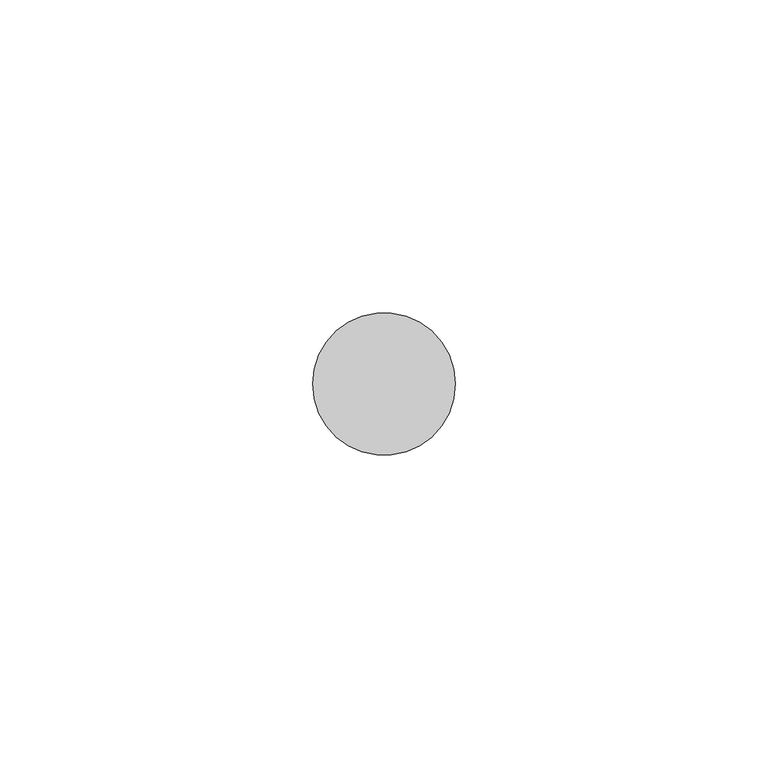
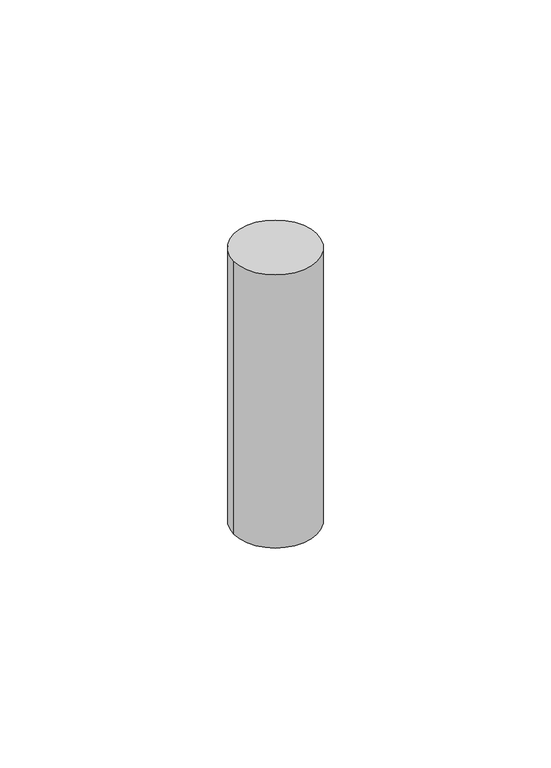
"""IFC4 building model written with IfcOpenShell, lengths in millimetres: proxy geometry, Bolt17:Bolt003:304645 : Bolt17:Bolt003:304645."""

from ifc_helpers import new_model, si_unit, point, frame, frame_2d, origin, place, context, project, spatial, circle_curve, trimmed, segment, composite_curve, outline, extrude, source, transform, mapped, element, save


def generic_models_3cd3809d(model_context):
    return source(origin(), model_context, "Body", "SweptSolid", [
        extrude(outline(composite_curve([segment(trimmed(circle_curve(frame_2d((9949.3919204, 2276.5207483)), 11.4045168), [point((9937.9874035, 2276.5207483))], [point((9960.7964372, 2276.5207483))], False, "CARTESIAN"), True, "CONTINUOUS"), segment(trimmed(circle_curve(frame_2d((9949.3919204, 2276.5207483)), 11.4045168), [point((9960.7964372, 2276.5207483))], [point((9937.9874035, 2276.5207483))], False, "CARTESIAN"), True, "CONTINUOUS")], self_intersect=False)), frame((0.0, 0.0, 36645.5959962), z_axis=(0.0, 0.0, 1.0), x_axis=(1.0, 0.0, 0.0)), (0.0, 0.0, 1.0), 79.375),
    ])


if __name__ == "__main__":
    model = new_model("IFC4")
    model_context = context("Model", 3, world=origin())
    ifc_project = project(units=[si_unit("LENGTHUNIT", "METRE", prefix="MILLI")], contexts=[model_context])
    site = spatial("IfcSite", under=ifc_project)
    building = spatial("IfcBuilding", under=site)
    placement = place(None, origin())
    generic_models_shape = generic_models_3cd3809d(model_context)
    element("IfcBuildingElementProxy", 1, Name="Bolt17:Bolt003:304645 : Bolt17:Bolt003:304645", ObjectType="Bolt17:Bolt003:304645 : Bolt17:Bolt003:304645", at=placement, inside=building, context=model_context, shape_type="MappedRepresentation", body=[
        mapped(generic_models_shape, transform((0.0, 0.0, 0.0), x_axis=(1.0, 0.0, 0.0), y_axis=(0.0, 1.0, 0.0), z_axis=(0.0, 0.0, 1.0))),
    ])
    save(model, "model.ifc")

# Revit data of these elements
# Type "Bolt17:Bolt003:304645 : Bolt17:Bolt003:304645"
#   NameOverride = "Bolt17:Bolt003:304645"
#   ObjectTypeOverride = "Bolt17:Bolt003"
#   Reference = "Bolt003"
#   Category = "Generic Models"
#   Tag = "304645"
# Element 1 (IfcBuildingElementProxy, "Bolt17:Bolt003:304645 : Bolt17:Bolt003:304645")
#   Materials on its faces: "TUBE STEEL STRINGER WELDED TO ANCHORED STEEL PLATE - SEE STRUCT DWGS"
# Materials
#   "TUBE STEEL STRINGER WELDED TO ANCHORED STEEL PLATE - SEE STRUCT DWGS": class "Unassigned", colour RGB 128 128 128, transparency 0, Cost = 0
